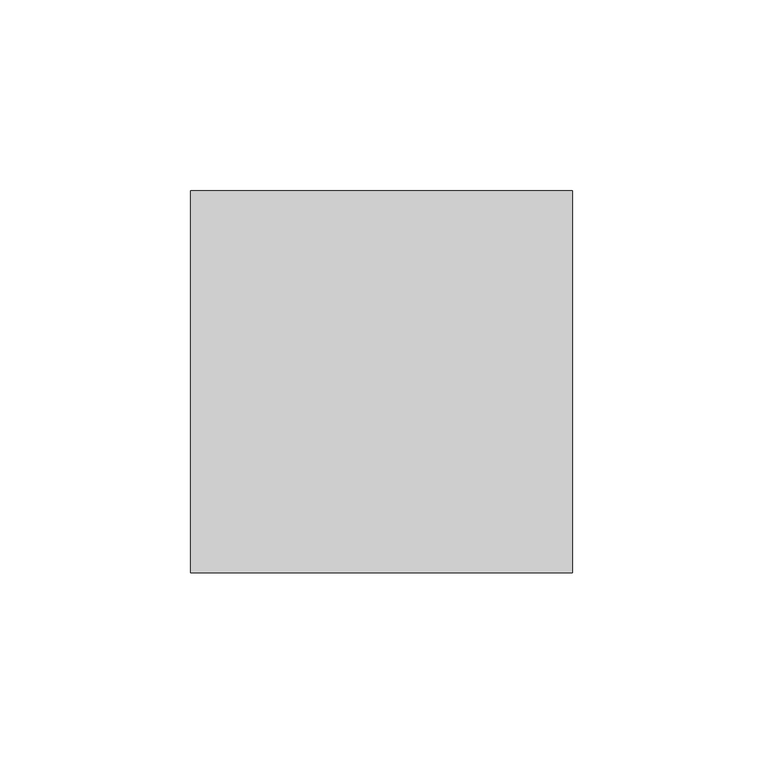
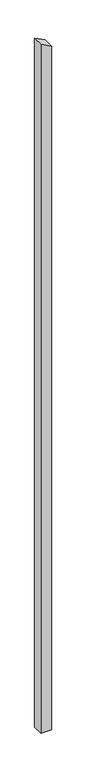
"""IFC4 building model written with IfcOpenShell, lengths in millimetres: column geometry, Holzstütze 158956 : Holzstütze 158956."""

from ifc_helpers import new_model, si_unit, frame, origin, place, context, project, spatial, polyline, outline, extrude, source, transform, mapped, element, save


def column_af1205e1(model_context):
    return source(origin(), model_context, "Body", "SweptSolid", [
        extrude(outline(polyline([(-500.0, 174197.7593015), (-500.0, 174297.7593015), (6345.7118258, 174297.7593015), (6396.6643707, 174197.7593015), (-500.0, 174197.7593015)])), frame((0.0, 26981.9343946, 0.0), z_axis=(0.0, 1.0, 0.0), x_axis=(0.0, 0.0, 1.0)), (0.0, 0.0, 1.0), 100.0),
    ])


if __name__ == "__main__":
    model = new_model("IFC4")
    model_context = context("Model", 3, world=origin())
    ifc_project = project(units=[si_unit("LENGTHUNIT", "METRE", prefix="MILLI")], contexts=[model_context])
    site = spatial("IfcSite", under=ifc_project)
    building = spatial("IfcBuilding", under=site)
    placement = place(None, origin())
    column_shape = column_af1205e1(model_context)
    element("IfcColumn", 1, ObjectType="Holzstütze 158956 : Holzstütze 158956", at=placement, inside=building, context=model_context, shape_type="MappedRepresentation", body=[
        mapped(column_shape, transform((0.0, 0.0, 0.0), x_axis=(1.0, 0.0, 0.0), y_axis=(0.0, 1.0, 0.0), z_axis=(0.0, 0.0, 1.0))),
    ])
    save(model, "model.ifc")

# Revit data of these elements
# Type "Holzstütze 158956 : Holzstütze 158956"
#   Abrechnungsart = "m"
#   Allright_Bauteil_ID = "0152St 0000143352"
#   Bezeichnung = "Holzstütze"
#   Codetext = "ST-HOLZ\\"
#   Gewerk = "Zimmer- und Holzbauarbeiten"
#   Material = "Holz"
#   Objektname = "Stütze"
#   NameOverride = "Holzstütze"
#   Reference = "Holzstütze"
#   Status = "NEW"
#   ThermalTransmittance = 0.0000 BTU/(h·ft²·°F)
#   Roll = 0.00°
#   Slope = 0.00°
#   2D Interaktion = yes
#   IsExternal = yes
#   LoadBearing = yes
# Element 1 (IfcColumn, "Holzstütze 158956 : Holzstütze 158956")
#   Materials on its faces: "holzschalung"
# Materials
#   "holzschalung": class "Unassigned", colour RGB 128 128 128, transparency 0
